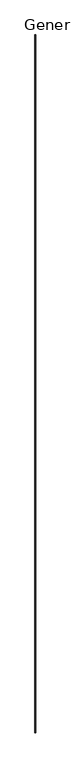
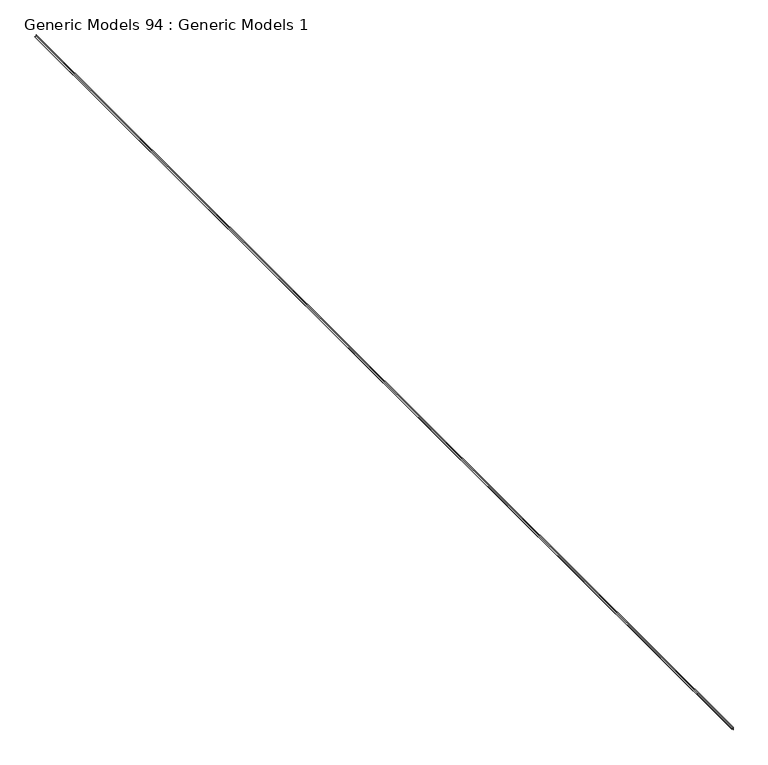
"""IFC4 building model written with IfcOpenShell, lengths in millimetres: proxy geometry, Generic Models 94 : Generic Models 1."""

from ifc_helpers import new_model, si_unit, frame, origin, place, context, project, spatial, polyline, outline, extrude, source, transform, mapped, element, save


def generic_models_94_generic_models_1_dbaa7c81(model_context):
    return source(origin(), model_context, "Body", "SweptSolid", [
        extrude(outline(polyline([(126375.541, -8999.7331401), (126375.541, -9001.0031401), (126356.491, -9001.0031401), (126356.491, -9021.9581401), (126351.7412, -9021.9581401), (126351.7412, -9020.6881401), (126355.221, -9020.6881401), (126355.221, -9001.0031401), (126336.171, -9001.0031401), (126336.171, -8999.7331401), (126375.541, -8999.7331401)])), frame((0.0, -7068.1230338, 0.0), z_axis=(0.0, 1.0, 0.0), x_axis=(0.0, 0.0, 1.0)), (0.0, 0.0, 1.0), 19050.0),
    ])


if __name__ == "__main__":
    model = new_model("IFC4")
    model_context = context("Model", 3, world=origin())
    ifc_project = project(units=[si_unit("LENGTHUNIT", "METRE", prefix="MILLI")], contexts=[model_context])
    site = spatial("IfcSite", under=ifc_project)
    building = spatial("IfcBuilding", under=site)
    placement = place(None, origin())
    generic_models_94_generic_models_1_shape = generic_models_94_generic_models_1_dbaa7c81(model_context)
    element("IfcBuildingElementProxy", 1, Name="Generic Models 94 : Generic Models 1", ObjectType="Generic Models 94 : Generic Models 1", at=placement, inside=building, context=model_context, shape_type="MappedRepresentation", body=[
        mapped(generic_models_94_generic_models_1_shape, transform((0.0, 0.0, 0.0), x_axis=(1.0, 0.0, 0.0), y_axis=(0.0, 1.0, 0.0), z_axis=(0.0, 0.0, 1.0))),
    ])
    save(model, "model.ifc")

# Revit data of these elements
# Element 1 (IfcBuildingElementProxy, "Generic Models 94 : Generic Models 1")
#   Materials on its faces: "_ 16 GA. COPPER VENTED T REVEAL BEAD (CONT. AROUND PERIMETER OF BEAM)"
# Materials
#   "_ 16 GA. COPPER VENTED T REVEAL BEAD (CONT. AROUND PERIMETER OF BEAM)": class "Generic", colour RGB 253 192 103, transparency 0, Cost = 0
